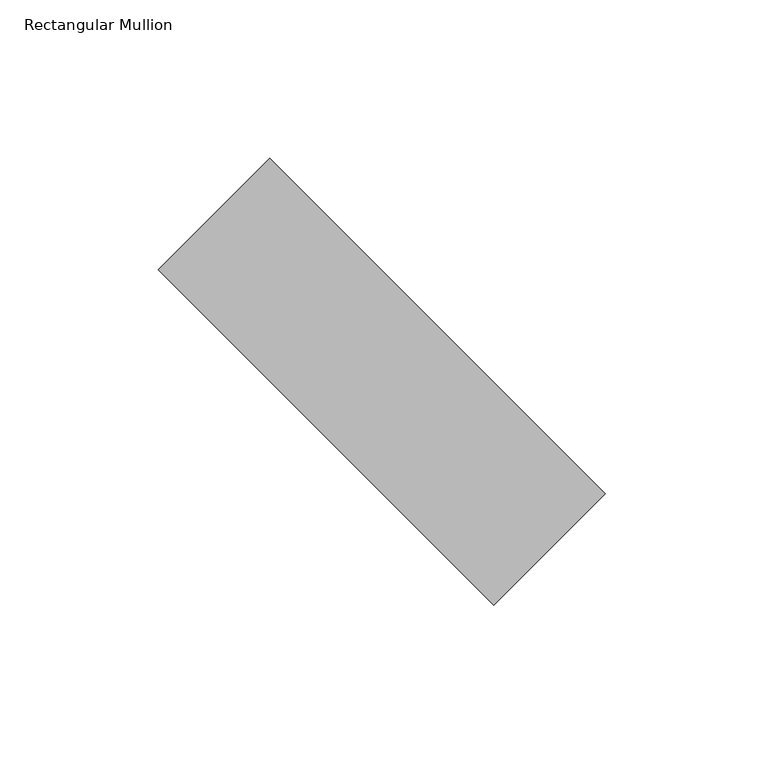
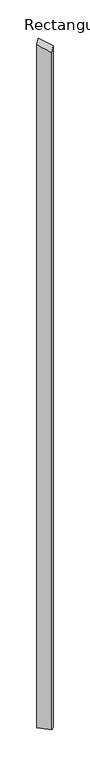
"""IFC4 building model written with IfcOpenShell, lengths in millimetres: member geometry, Rectangular Mullion : tilted mullions."""

import ifcopenshell
import ifcopenshell.guid

model = None  # the IFC model being written
_history = None  # IfcOwnerHistory: only IFC2X3 demands one
_inside = {}  # id of a spatial element -> (the spatial element, [elements in it])
_under = {}  # id of a project, library or spatial element -> (it, [spatial elements below it])
_declared = {}  # id of a project -> (the project, [libraries it declares])
_typed = {}  # id of a type object -> (the type object, [elements of that type])
_made_of = {}  # id of a material, layer set ... -> (it, [elements and type objects made of it])


def new_model(schema):
    """Start an empty IFC model of exactly this schema.

    Asked for "IFC4X3", IfcOpenShell would pick the latest addendum, in which some entities
    have other attributes; the version numbers below select the first issue.
    IFC2X3 requires an IfcOwnerHistory on every rooted entity: one is made here for all.
    """
    global model, _history
    if schema == "IFC4X3":
        model = ifcopenshell.file(schema_version=(4, 3, 0, 0))
    else:
        model = ifcopenshell.file(schema=schema)
    _inside.clear()
    _under.clear()
    _declared.clear()
    _typed.clear()
    _made_of.clear()
    _history = None
    if model.schema == "IFC2X3":
        org = make("IfcOrganization", Name="unknown")
        user = make(
            "IfcPersonAndOrganization",
            ThePerson=make("IfcPerson", FamilyName="unknown"),
            TheOrganization=org,
        )
        app = make(
            "IfcApplication",
            ApplicationDeveloper=org,
            Version="unknown",
            ApplicationFullName="unknown",
            ApplicationIdentifier="unknown",
        )
        _history = make(
            "IfcOwnerHistory",
            OwningUser=user,
            OwningApplication=app,
            ChangeAction="ADDED",
            CreationDate=0,
        )
    return model


def make(cls, **values):
    """One entity of the class cls with the attributes given. An attribute that is None is left unset."""
    return model.create_entity(
        cls, **{name: value for name, value in values.items() if value is not None}
    )


def rooted(cls, **values):
    """An entity with a GlobalId (a new one), such as an element, a storey or a relation."""
    return make(cls, GlobalId=ifcopenshell.guid.new(), OwnerHistory=_history, **values)


def si_unit(unit_type, name, prefix=None):
    """IfcSIUnit, for example si_unit("LENGTHUNIT", "METRE", prefix="MILLI")."""
    return make("IfcSIUnit", UnitType=unit_type, Prefix=prefix, Name=name)


def assignment(units):
    """IfcUnitAssignment: the units of a project."""
    return None if units is None else make("IfcUnitAssignment", Units=units)


def point(xyz):
    """IfcCartesianPoint."""
    return None if xyz is None else make("IfcCartesianPoint", Coordinates=xyz)


def direction(xyz):
    """IfcDirection."""
    return None if xyz is None else make("IfcDirection", DirectionRatios=xyz)


def frame(location, z_axis=None, x_axis=None):
    """IfcAxis2Placement3D, a coordinate frame: its origin and axes. An axis left out is left unset."""
    return make(
        "IfcAxis2Placement3D",
        Location=point(location),
        Axis=direction(z_axis),
        RefDirection=direction(x_axis),
    )


def origin():
    """The frame at (0, 0, 0) with its axes left unset."""
    return frame((0.0, 0.0, 0.0))


def place(relative_to, where):
    """IfcLocalPlacement: puts the frame where relative to a parent placement (None: the world)."""
    return make(
        "IfcLocalPlacement", PlacementRelTo=relative_to, RelativePlacement=where
    )


def context(
    kind, dimensions, precision=None, world=None, true_north=None, identifier=None
):
    """IfcGeometricRepresentationContext, for example the 3D "Model" context."""
    return make(
        "IfcGeometricRepresentationContext",
        ContextIdentifier=identifier,
        ContextType=kind,
        CoordinateSpaceDimension=dimensions,
        Precision=precision,
        WorldCoordinateSystem=world,
        TrueNorth=true_north,
    )


def project(units=None, contexts=None):
    """IfcProject with its units and contexts."""
    return rooted(
        "IfcProject",
        Name="project",
        RepresentationContexts=contexts,
        UnitsInContext=assignment(units),
    )


def spatial(cls, under=None, at=None, **own):
    """A site, building, storey or space (cls), placed at a placement, below another one or the project."""
    s = rooted(cls, ObjectPlacement=at, **own)
    if under is not None:
        _under.setdefault(under.id(), (under, []))[1].append(s)
    return s


def faces_of(points, faces, orient=None, outer=None):
    """IfcFace entities. A face is a list of loops; a loop is a list of indices into points, from 0.

    orient and outer hold one flag for each loop. By default every Orientation is true, the
    first loop of a face is its IfcFaceOuterBound and the others are IfcFaceBound.
    """
    made = []
    for i, loops in enumerate(faces):
        bounds = []
        for j, loop in enumerate(loops):
            is_outer = j == 0 if outer is None else outer[i][j]
            bounds.append(
                make(
                    "IfcFaceOuterBound" if is_outer else "IfcFaceBound",
                    Bound=make("IfcPolyLoop", Polygon=[points[k] for k in loop]),
                    Orientation=True if orient is None else orient[i][j],
                )
            )
        made.append(make("IfcFace", Bounds=bounds))
    return made


def faceted_brep(points, faces, orient=None, outer=None, voids=None):
    """IfcFacetedBrep: a solid bounded by flat faces; with voids (closed shells), ...WithVoids."""
    shared = [point(p) for p in points]
    hull = make("IfcClosedShell", CfsFaces=faces_of(shared, faces, orient, outer))
    if voids is None:
        return make("IfcFacetedBrep", Outer=hull)
    return make(
        "IfcFacetedBrepWithVoids",
        Outer=hull,
        Voids=[
            make(cls, CfsFaces=faces_of(shared, fs, o, b)) for cls, fs, o, b in voids
        ],
    )


def shape(context_of_items, identifier, shape_type, items):
    """IfcShapeRepresentation: the items that make up one representation, for example the "Body"."""
    return make(
        "IfcShapeRepresentation",
        ContextOfItems=context_of_items,
        RepresentationIdentifier=identifier,
        RepresentationType=shape_type,
        Items=items,
    )


def source(mapping_origin, context_of_items, identifier, shape_type, items):
    """IfcRepresentationMap: a shape defined once, which mapped items show again and again."""
    return make(
        "IfcRepresentationMap",
        MappingOrigin=mapping_origin,
        MappedRepresentation=shape(context_of_items, identifier, shape_type, items),
    )


def transform(
    local_origin,
    x_axis=None,
    y_axis=None,
    z_axis=None,
    scale=None,
    scale2=None,
    scale3=None,
    uniform=True,
):
    """IfcCartesianTransformationOperator3D, or its non-uniform kind. x_axis, y_axis, z_axis: its Axis1, 2, 3."""
    if uniform:
        return make(
            "IfcCartesianTransformationOperator3D",
            Axis1=direction(x_axis),
            Axis2=direction(y_axis),
            LocalOrigin=point(local_origin),
            Scale=scale,
            Axis3=direction(z_axis),
        )
    return make(
        "IfcCartesianTransformationOperator3DnonUniform",
        Axis1=direction(x_axis),
        Axis2=direction(y_axis),
        LocalOrigin=point(local_origin),
        Scale=scale,
        Axis3=direction(z_axis),
        Scale2=scale2,
        Scale3=scale3,
    )


def mapped(mapping_source, mapping_target):
    """IfcMappedItem: shows the shape of a source again, moved by a transform."""
    return make(
        "IfcMappedItem", MappingSource=mapping_source, MappingTarget=mapping_target
    )


def made_of(thing, what):
    """Note that an element or type object is made of a material, layer set ...; save() writes the relation."""
    if what is not None:
        _made_of.setdefault(what.id(), (what, []))[1].append(thing)
    return thing


def element(
    cls,
    number,
    at=None,
    inside=None,
    cuts=None,
    type_object=None,
    material=None,
    context=None,
    identifier="Body",
    shape_type=None,
    held_by="IfcProductDefinitionShape",
    body=None,
    shapes=None,
    **own,
):
    """One element of the class cls, such as IfcWall. Its Tag is "e" and its number.

    at: its placement. inside: the storey or other place that contains it. cuts: it is an
    opening in that element (IfcRelVoidsElement). A single representation is given by context,
    identifier, shape_type and body (its items); several are given by shapes. held_by: the class
    of the entity that holds the representations. save() writes the other relations.
    """
    e = rooted(cls, Tag="e%d" % number, ObjectPlacement=at, **own)
    if body is not None:
        shapes = [shape(context, identifier, shape_type, body)]
    if shapes is not None:
        e.Representation = make(held_by, Representations=shapes)
    if inside is not None:
        _inside.setdefault(inside.id(), (inside, []))[1].append(e)
    if cuts is not None:
        rooted(
            "IfcRelVoidsElement", RelatingBuildingElement=cuts, RelatedOpeningElement=e
        )
    if type_object is not None:
        _typed.setdefault(type_object.id(), (type_object, []))[1].append(e)
    return made_of(e, material)


def aggregate(whole, parts):
    """IfcRelAggregates: a whole, such as a stair, and the parts it consists of."""
    return rooted("IfcRelAggregates", RelatingObject=whole, RelatedObjects=parts)


def save(model, path):
    """Write the relations noted so far, then the file.

    IfcRelAggregates (storeys below a building ...), IfcRelContainedInSpatialStructure (elements
    in a storey), IfcRelDefinesByType, IfcRelAssociatesMaterial and IfcRelDeclares: one each for
    every whole, place, type object, material and project.
    """
    for whole, parts in _under.values():
        aggregate(whole, parts)
    for where, things in _inside.values():
        rooted(
            "IfcRelContainedInSpatialStructure",
            RelatedElements=things,
            RelatingStructure=where,
        )
    for kind, things in _typed.values():
        rooted("IfcRelDefinesByType", RelatedObjects=things, RelatingType=kind)
    for what, things in _made_of.values():
        rooted("IfcRelAssociatesMaterial", RelatedObjects=things, RelatingMaterial=what)
    for by, libraries in _declared.values():
        rooted("IfcRelDeclares", RelatingContext=by, RelatedDefinitions=libraries)
    model.write(path)


def rectangular_mullion_824f0a5b(model_context):
    return source(origin(), model_context, "Body", "Brep", [
        faceted_brep([(-35.3553391, 70.7106781, -7999.8696296), (70.7106781, -35.3553391, -7999.8696296), (35.3553391, -70.7106781, -7999.8696296), (-70.7106781, 35.3553391, -7999.8696296), (-70.7106781, 35.3553391, 9.9721072), (-35.3553391, 70.7106781, 55.0329782), (35.3553391, -70.7106781, -55.0329782), (70.7106781, -35.3553391, -9.9721072)], [[[0, 1, 2, 3]], [[4, 5, 0, 3]], [[6, 4, 3, 2]], [[7, 6, 2, 1]], [[5, 7, 1, 0]], [[5, 4, 6, 7]]]),
    ])


if __name__ == "__main__":
    model = new_model("IFC4")
    model_context = context("Model", 3, world=origin())
    ifc_project = project(units=[si_unit("LENGTHUNIT", "METRE", prefix="MILLI")], contexts=[model_context])
    site = spatial("IfcSite", under=ifc_project)
    building = spatial("IfcBuilding", under=site)
    placement = place(None, origin())
    rectangular_mullion_shape = rectangular_mullion_824f0a5b(model_context)
    element("IfcMember", 1, ObjectType="Rectangular Mullion : tilted mullions", at=placement, inside=building, context=model_context, shape_type="MappedRepresentation", body=[
        mapped(rectangular_mullion_shape, transform((0.0, 0.0, 0.0), x_axis=(1.0, 0.0, 0.0), y_axis=(0.0, 1.0, 0.0), z_axis=(0.0, 0.0, 1.0))),
    ])
    save(model, "model.ifc")

# Revit data of these elements
# Type "Rectangular Mullion : tilted mullions"
#   built-in parameter 1007304 = 0.492126 (stored number, unit not read)
#   built-in parameter 1007301 = 0.082021 (stored number, unit not read)
#   built-in parameter 1007300 = 0.082021 (stored number, unit not read)
# Element 1 (IfcMember, "Rectangular Mullion : tilted mullions")
#   Materials on its faces: "Aluminum"
# Materials
#   "Aluminum": class "Metal", colour RGB 244 244 244, transparency 0, Description = "Aluminum 6061", Cost = 0
